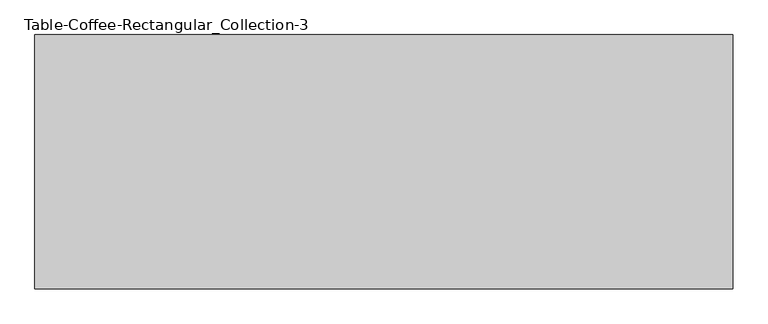
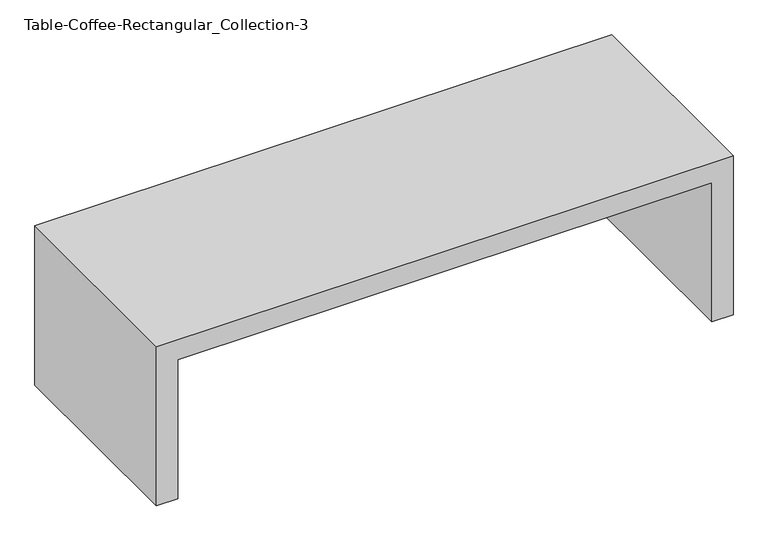
"""IFC4 building model written with IfcOpenShell, lengths in millimetres: furniture geometry, _Produtos_Arq_Bib_Table-Coffee-Rectangular_Collection-3_Reed : Table-Coffee-Rectangular_Collection-3."""

from ifc_helpers import new_model, si_unit, frame, origin, place, context, project, spatial, polyline, outline, extrude, source, transform, mapped, element, save


def table_coffee_rectangular_collection_3_aec037ed(model_context):
    return source(origin(), model_context, "Body", "SweptSolid", [
        extrude(outline(polyline([(0.0, -685.8), (0.0, -635.0), (349.2, -635.0), (349.2, 635.0), (0.0, 635.0), (0.0, 685.8), (400.0, 685.8), (400.0, -685.8), (0.0, -685.8)])), frame((0.0, -250.0, 0.0), z_axis=(0.0, 1.0, 0.0), x_axis=(0.0, 0.0, 1.0)), (0.0, 0.0, 1.0), 500.0),
    ])


if __name__ == "__main__":
    model = new_model("IFC4")
    model_context = context("Model", 3, world=origin())
    ifc_project = project(units=[si_unit("LENGTHUNIT", "METRE", prefix="MILLI")], contexts=[model_context])
    site = spatial("IfcSite", under=ifc_project)
    building = spatial("IfcBuilding", under=site)
    placement = place(None, origin())
    table_coffee_rectangular_collection_3_shape = table_coffee_rectangular_collection_3_aec037ed(model_context)
    element("IfcFurniture", 1, ObjectType="_Produtos_Arq_Bib_Table-Coffee-Rectangular_Collection-3_Reed : Table-Coffee-Rectangular_Collection-3", at=placement, inside=building, context=model_context, shape_type="MappedRepresentation", body=[
        mapped(table_coffee_rectangular_collection_3_shape, transform((0.0, 0.0, 0.0), x_axis=(1.0, 0.0, 0.0), y_axis=(0.0, 1.0, 0.0), z_axis=(0.0, 0.0, 1.0))),
    ])
    save(model, "model.ifc")

# Revit data of these elements
# Type "_Produtos_Arq_Bib_Table-Coffee-Rectangular_Collection-3_Reed : Table-Coffee-Rectangular_Collection-3"
#   Subcategory = "Table\r\n"
#   SmartBIM Object Created By = "Reed Construction Data"
#   Assembly Code = "E2020200"
#   95 CSI = "12584"
#   04 CSI = "16 58 23"
#   Width = 1.3716 m
#   SmartBIM Object Version = 3
#   Offset = 0.0508 m
#   Height = 0.4 m
#   Depth = 0.5 m
#   Wood = Wood Cherry
#   Manufacturer = ""
#   Default Elevation = 0
# Element 1 (IfcFurniture, "_Produtos_Arq_Bib_Table-Coffee-Rectangular_Collection-3_Reed : Table-Coffee-Rectangular_Collection-3")
#   Materials on its faces: "Wood Cherry"
# Materials
#   "Wood Cherry": class "Unassigned", colour RGB 185 153 118, transparency 0
